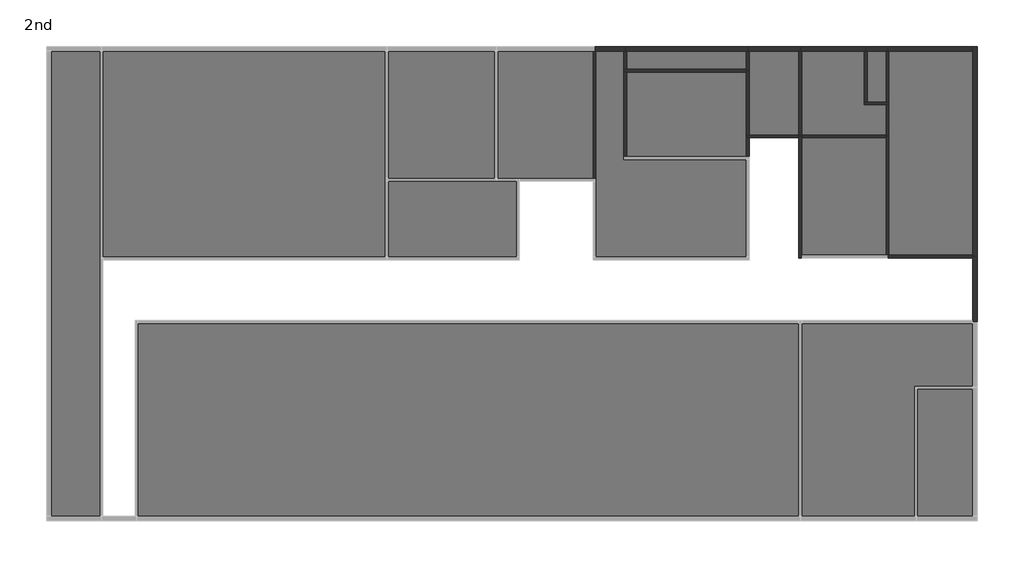
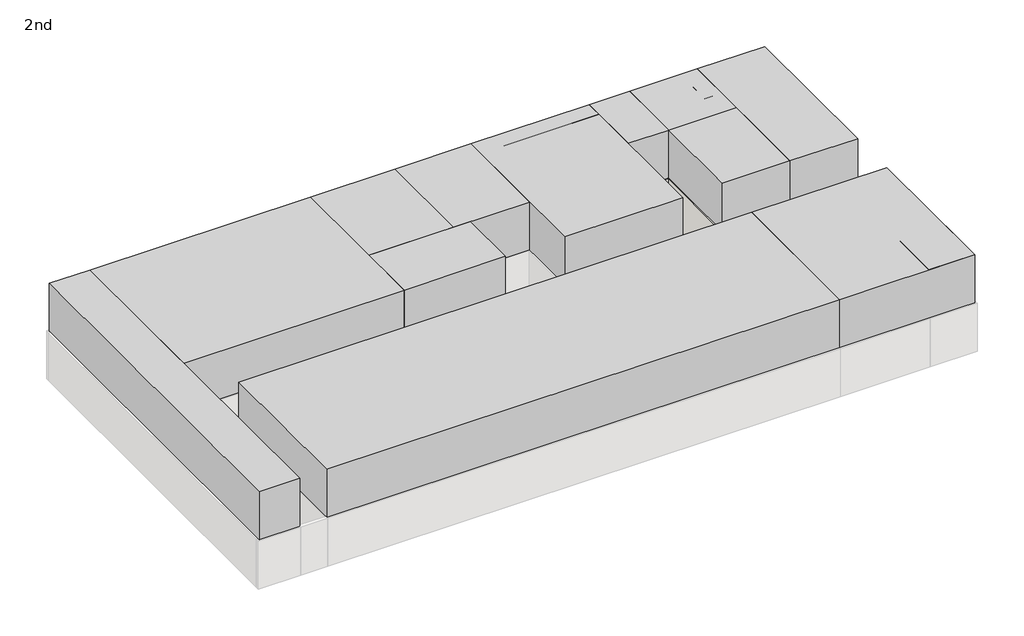
# One storey, part 2 of 2: 42 walls, 17 proxies.
# Revit data of these elements (continued)
# Element 14 (IfcBuildingElementProxy, "Space Planning Box : Space Planning Box") (continued)
#   Program Area = 31.5 m²
#   Length = 4000 mm
#   Height = 6000 mm
#   Area = 9.6 m²
#   Fill Color = Lavender
#   Phase Created = New Construction
#   Materials on its faces: "Lavender"
# Element 15 (IfcBuildingElementProxy, "Space Planning Box : Space Planning Box")
#   Room Name = "Locker Room (F)"
#   Width = 2400 mm
#   Program Area = 31.5 m²
#   Length = 4000 mm
#   Height = 6000 mm
#   Area = 9.6 m²
#   Fill Color = Lavender
#   Phase Created = New Construction
#   Materials on its faces: "Lavender"
# Element 16 (IfcBuildingElementProxy, "Space Planning Box : Space Planning Box")
#   Room Name = "Shower Room (M)"
#   Width = 1000 mm
#   Program Area = 31.5 m²
#   Length = 5600 mm
#   Height = 6000 mm
#   Area = 5.6 m²
#   Fill Color = Lavender
#   Phase Created = New Construction
#   Materials on its faces: "Lavender"
# Element 17 (IfcBuildingElementProxy, "Space Planning Box : Space Planning Box")
#   Room Name = "Locker Room (M)"
#   Width = 5600 mm
#   Program Area = 31.5 m²
#   Length = 5000 mm
#   Height = 6000 mm
#   Area = 28 m²
#   Fill Color = Lavender
#   Phase Created = New Construction
#   Materials on its faces: "Lavender"
# Elements 18, 19, 20, 21, 22, 23, 24, 25 (IfcWall, "Wall-Ext_215Bwk")
#   Top Offset = 0 mm
#   Base Offset = 0 mm
#   Unconnected Height = 3000 mm
#   wall height = 3000 mm
#   Phase Created = New Construction
#   Base Constraint = 2nd
#   Materials on its faces: "Brick, Common"
# Elements 26, 28, 29, 30, 31, 32, 33, 34, 35, 37, 38, 40, 41, 42, 43, 44, 46, 47, 48, 49, 51, 52, 53, 55, 56, 59 (IfcWall, "Wall-Int_12P-100Blk-12P")
#   Top Offset = 0 mm
#   Base Offset = 0 mm
#   Unconnected Height = 3000 mm
#   wall height = 3000 mm
#   Phase Created = New Construction
#   Base Constraint = 2nd
#   Materials on its faces: "Default Wall", "Plaster"
# Elements 27, 36, 39, 45, 50, 54, 57, 58 (IfcWall, "Wall-Int_12P-100Blk-12P")
#   Top Offset = 0 mm
#   Base Offset = 0 mm
#   Unconnected Height = 3000 mm
#   wall height = 3000 mm
#   Phase Created = New Construction
#   Base Constraint = 2nd
#   Materials on its faces: "Plaster", "Default Wall"
# Materials
#   "Cyan": class "Generic", colour RGB 0 255 255, transparency 0.2, Cost = 0
#   "Brick, Common": class "Masonry", colour RGB 170 100 105, transparency 0, Description = "Common brick", Cost = 0
#   "Plaster": class "Generic", colour RGB 249 249 249, transparency 0, Description = "Plaster", Cost = 0
#   "Concrete Masonry Units": class "Masonry", colour RGB 181 181 181, transparency 0, Description = "Concrete masonry units", Cost = 0
#   "Pink": class "Generic", colour RGB 255 105 180, transparency 0.2, Cost = 0
#   "Lime": class "Generic", colour RGB 0 255 0, transparency 0.2, Cost = 0
#   "Lavender": class "Generic", colour RGB 186 85 211, transparency 0.2, Cost = 0
#   "Default Wall": class "Miscellaneous", colour RGB 128 128 128, transparency 0, Comments = "Rendering appearance not upgraded Rendering appearance not upgraded ", Cost = 0
